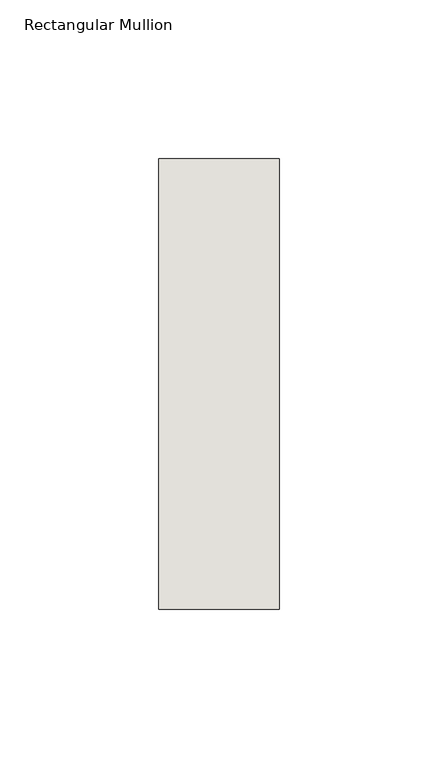
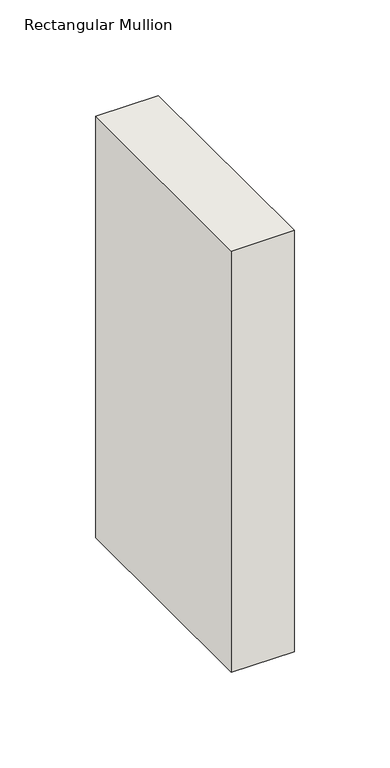
"""IFC4 building model written with IfcOpenShell, lengths in millimetres: wall geometry, Rectangular Mullion : NLRS_21_CWM_hsb-regel 38x142_gen_rsf."""

import ifcopenshell
import ifcopenshell.guid

model = None  # the IFC model being written
_history = None  # IfcOwnerHistory: only IFC2X3 demands one
_inside = {}  # id of a spatial element -> (the spatial element, [elements in it])
_under = {}  # id of a project, library or spatial element -> (it, [spatial elements below it])
_declared = {}  # id of a project -> (the project, [libraries it declares])
_typed = {}  # id of a type object -> (the type object, [elements of that type])
_made_of = {}  # id of a material, layer set ... -> (it, [elements and type objects made of it])


def new_model(schema):
    """Start an empty IFC model of exactly this schema.

    Asked for "IFC4X3", IfcOpenShell would pick the latest addendum, in which some entities
    have other attributes; the version numbers below select the first issue.
    IFC2X3 requires an IfcOwnerHistory on every rooted entity: one is made here for all.
    """
    global model, _history
    if schema == "IFC4X3":
        model = ifcopenshell.file(schema_version=(4, 3, 0, 0))
    else:
        model = ifcopenshell.file(schema=schema)
    _inside.clear()
    _under.clear()
    _declared.clear()
    _typed.clear()
    _made_of.clear()
    _history = None
    if model.schema == "IFC2X3":
        org = make("IfcOrganization", Name="unknown")
        user = make(
            "IfcPersonAndOrganization",
            ThePerson=make("IfcPerson", FamilyName="unknown"),
            TheOrganization=org,
        )
        app = make(
            "IfcApplication",
            ApplicationDeveloper=org,
            Version="unknown",
            ApplicationFullName="unknown",
            ApplicationIdentifier="unknown",
        )
        _history = make(
            "IfcOwnerHistory",
            OwningUser=user,
            OwningApplication=app,
            ChangeAction="ADDED",
            CreationDate=0,
        )
    return model


def make(cls, **values):
    """One entity of the class cls with the attributes given. An attribute that is None is left unset."""
    return model.create_entity(
        cls, **{name: value for name, value in values.items() if value is not None}
    )


def rooted(cls, **values):
    """An entity with a GlobalId (a new one), such as an element, a storey or a relation."""
    return make(cls, GlobalId=ifcopenshell.guid.new(), OwnerHistory=_history, **values)


def si_unit(unit_type, name, prefix=None):
    """IfcSIUnit, for example si_unit("LENGTHUNIT", "METRE", prefix="MILLI")."""
    return make("IfcSIUnit", UnitType=unit_type, Prefix=prefix, Name=name)


def assignment(units):
    """IfcUnitAssignment: the units of a project."""
    return None if units is None else make("IfcUnitAssignment", Units=units)


def point(xyz):
    """IfcCartesianPoint."""
    return None if xyz is None else make("IfcCartesianPoint", Coordinates=xyz)


def direction(xyz):
    """IfcDirection."""
    return None if xyz is None else make("IfcDirection", DirectionRatios=xyz)


def frame(location, z_axis=None, x_axis=None):
    """IfcAxis2Placement3D, a coordinate frame: its origin and axes. An axis left out is left unset."""
    return make(
        "IfcAxis2Placement3D",
        Location=point(location),
        Axis=direction(z_axis),
        RefDirection=direction(x_axis),
    )


def origin():
    """The frame at (0, 0, 0) with its axes left unset."""
    return frame((0.0, 0.0, 0.0))


def place(relative_to, where):
    """IfcLocalPlacement: puts the frame where relative to a parent placement (None: the world)."""
    return make(
        "IfcLocalPlacement", PlacementRelTo=relative_to, RelativePlacement=where
    )


def context(
    kind, dimensions, precision=None, world=None, true_north=None, identifier=None
):
    """IfcGeometricRepresentationContext, for example the 3D "Model" context."""
    return make(
        "IfcGeometricRepresentationContext",
        ContextIdentifier=identifier,
        ContextType=kind,
        CoordinateSpaceDimension=dimensions,
        Precision=precision,
        WorldCoordinateSystem=world,
        TrueNorth=true_north,
    )


def project(units=None, contexts=None):
    """IfcProject with its units and contexts."""
    return rooted(
        "IfcProject",
        Name="project",
        RepresentationContexts=contexts,
        UnitsInContext=assignment(units),
    )


def spatial(cls, under=None, at=None, **own):
    """A site, building, storey or space (cls), placed at a placement, below another one or the project."""
    s = rooted(cls, ObjectPlacement=at, **own)
    if under is not None:
        _under.setdefault(under.id(), (under, []))[1].append(s)
    return s


def polyline(points):
    """IfcPolyline through the points."""
    return make("IfcPolyline", Points=[point(p) for p in points])


def outline(outer, holes=None, kind="AREA"):
    """IfcArbitraryClosedProfileDef: a profile drawn as a closed curve; with holes, ...WithVoids."""
    if holes is None:
        return make("IfcArbitraryClosedProfileDef", ProfileType=kind, OuterCurve=outer)
    return make(
        "IfcArbitraryProfileDefWithVoids",
        ProfileType=kind,
        OuterCurve=outer,
        InnerCurves=holes,
    )


def extrude(swept, where, along, depth):
    """IfcExtrudedAreaSolid: the profile swept, set in the frame where, extruded along a direction by depth."""
    return make(
        "IfcExtrudedAreaSolid",
        SweptArea=swept,
        Position=where,
        ExtrudedDirection=direction(along),
        Depth=depth,
    )


def shape(context_of_items, identifier, shape_type, items):
    """IfcShapeRepresentation: the items that make up one representation, for example the "Body"."""
    return make(
        "IfcShapeRepresentation",
        ContextOfItems=context_of_items,
        RepresentationIdentifier=identifier,
        RepresentationType=shape_type,
        Items=items,
    )


def source(mapping_origin, context_of_items, identifier, shape_type, items):
    """IfcRepresentationMap: a shape defined once, which mapped items show again and again."""
    return make(
        "IfcRepresentationMap",
        MappingOrigin=mapping_origin,
        MappedRepresentation=shape(context_of_items, identifier, shape_type, items),
    )


def transform(
    local_origin,
    x_axis=None,
    y_axis=None,
    z_axis=None,
    scale=None,
    scale2=None,
    scale3=None,
    uniform=True,
):
    """IfcCartesianTransformationOperator3D, or its non-uniform kind. x_axis, y_axis, z_axis: its Axis1, 2, 3."""
    if uniform:
        return make(
            "IfcCartesianTransformationOperator3D",
            Axis1=direction(x_axis),
            Axis2=direction(y_axis),
            LocalOrigin=point(local_origin),
            Scale=scale,
            Axis3=direction(z_axis),
        )
    return make(
        "IfcCartesianTransformationOperator3DnonUniform",
        Axis1=direction(x_axis),
        Axis2=direction(y_axis),
        LocalOrigin=point(local_origin),
        Scale=scale,
        Axis3=direction(z_axis),
        Scale2=scale2,
        Scale3=scale3,
    )


def mapped(mapping_source, mapping_target):
    """IfcMappedItem: shows the shape of a source again, moved by a transform."""
    return make(
        "IfcMappedItem", MappingSource=mapping_source, MappingTarget=mapping_target
    )


def made_of(thing, what):
    """Note that an element or type object is made of a material, layer set ...; save() writes the relation."""
    if what is not None:
        _made_of.setdefault(what.id(), (what, []))[1].append(thing)
    return thing


def element(
    cls,
    number,
    at=None,
    inside=None,
    cuts=None,
    type_object=None,
    material=None,
    context=None,
    identifier="Body",
    shape_type=None,
    held_by="IfcProductDefinitionShape",
    body=None,
    shapes=None,
    **own,
):
    """One element of the class cls, such as IfcWall. Its Tag is "e" and its number.

    at: its placement. inside: the storey or other place that contains it. cuts: it is an
    opening in that element (IfcRelVoidsElement). A single representation is given by context,
    identifier, shape_type and body (its items); several are given by shapes. held_by: the class
    of the entity that holds the representations. save() writes the other relations.
    """
    e = rooted(cls, Tag="e%d" % number, ObjectPlacement=at, **own)
    if body is not None:
        shapes = [shape(context, identifier, shape_type, body)]
    if shapes is not None:
        e.Representation = make(held_by, Representations=shapes)
    if inside is not None:
        _inside.setdefault(inside.id(), (inside, []))[1].append(e)
    if cuts is not None:
        rooted(
            "IfcRelVoidsElement", RelatingBuildingElement=cuts, RelatedOpeningElement=e
        )
    if type_object is not None:
        _typed.setdefault(type_object.id(), (type_object, []))[1].append(e)
    return made_of(e, material)


def aggregate(whole, parts):
    """IfcRelAggregates: a whole, such as a stair, and the parts it consists of."""
    return rooted("IfcRelAggregates", RelatingObject=whole, RelatedObjects=parts)


def save(model, path):
    """Write the relations noted so far, then the file.

    IfcRelAggregates (storeys below a building ...), IfcRelContainedInSpatialStructure (elements
    in a storey), IfcRelDefinesByType, IfcRelAssociatesMaterial and IfcRelDeclares: one each for
    every whole, place, type object, material and project.
    """
    for whole, parts in _under.values():
        aggregate(whole, parts)
    for where, things in _inside.values():
        rooted(
            "IfcRelContainedInSpatialStructure",
            RelatedElements=things,
            RelatingStructure=where,
        )
    for kind, things in _typed.values():
        rooted("IfcRelDefinesByType", RelatedObjects=things, RelatingType=kind)
    for what, things in _made_of.values():
        rooted("IfcRelAssociatesMaterial", RelatedObjects=things, RelatingMaterial=what)
    for by, libraries in _declared.values():
        rooted("IfcRelDeclares", RelatingContext=by, RelatedDefinitions=libraries)
    model.write(path)


def rectangular_mullion_ffaa0eaf(model_context):
    return source(origin(), model_context, "Body", "SweptSolid", [
        extrude(outline(polyline([(0.0, -71.0), (-38.0, -71.0), (-38.0, 71.0), (0.0, 71.0), (0.0, -71.0)])), frame((0.0, 0.0, -269.0000003), z_axis=(0.0, 0.0, 1.0), x_axis=(1.0, 0.0, 0.0)), (0.0, 0.0, 1.0), 269.0000003),
    ])


if __name__ == "__main__":
    model = new_model("IFC4")
    model_context = context("Model", 3, world=origin())
    ifc_project = project(units=[si_unit("LENGTHUNIT", "METRE", prefix="MILLI")], contexts=[model_context])
    site = spatial("IfcSite", under=ifc_project)
    building = spatial("IfcBuilding", under=site)
    placement = place(None, origin())
    rectangular_mullion_shape = rectangular_mullion_ffaa0eaf(model_context)
    element("IfcWall", 1, ObjectType="Rectangular Mullion : NLRS_21_CWM_hsb-regel 38x142_gen_rsf", at=placement, inside=building, context=model_context, shape_type="MappedRepresentation", body=[
        mapped(rectangular_mullion_shape, transform((0.0, 0.0, 0.0), x_axis=(1.0, 0.0, 0.0), y_axis=(0.0, 1.0, 0.0), z_axis=(0.0, 0.0, 1.0))),
    ])
    save(model, "model.ifc")

# Revit data of these elements
# Type "Rectangular Mullion : NLRS_21_CWM_hsb-regel 38x142_gen_rsf"
#   Type IfcGUID = "07M7mRoiH1CR8m_RSKIwpF"
#   Assembly Code = "21.10"
#   IfcExportAs = "IfcWall"
#   built-in parameter 1007322 = 0.465879 (stored number, unit not read)
#   built-in parameter 1007321 = 0.062336 (stored number, unit not read)
#   built-in parameter 1007320 = 0.062336 (stored number, unit not read)
# Element 1 (IfcWall, "Rectangular Mullion : NLRS_21_CWM_hsb-regel 38x142_gen_rsf")
#   Materials on its faces: "NLRS_i2_hout naaldhout vuren_gen_rsf"
# Materials
#   "NLRS_i2_hout naaldhout vuren_gen_rsf": class "I - Hout", colour RGB 234 199 147, transparency 0, Keynote = "i2", Manufacturer = "Revit Standards Foundation", URL = "www.revitstandards.org", Description = "hout vuren", Cost = 0
